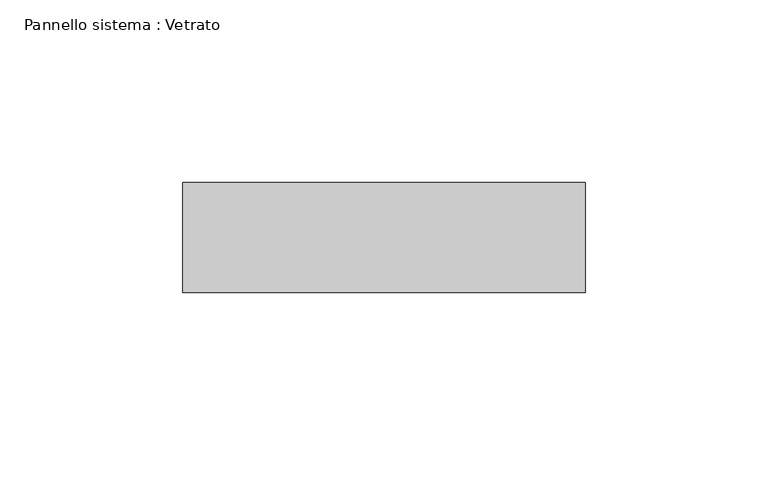
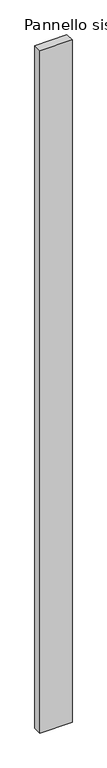
"""IFC4 building model written with IfcOpenShell, lengths in millimetres: plate geometry, Pannello sistema : Vetrato."""

from ifc_helpers import new_model, si_unit, origin, origin_with_axes, place, context, project, spatial, polyline, outline, extrude, source, transform, mapped, element, save


def pannello_sistema_vetrato_b6e2c1f0(model_context):
    return source(origin(), model_context, "Body", "SweptSolid", [
        extrude(outline(polyline([(55.0, -15.0), (-55.0, -15.0), (-55.0, 15.0), (55.0, 15.0), (55.0, -15.0)])), origin_with_axes(), (0.0, 0.0, 1.0), 2475.0),
    ])


if __name__ == "__main__":
    model = new_model("IFC4")
    model_context = context("Model", 3, world=origin())
    ifc_project = project(units=[si_unit("LENGTHUNIT", "METRE", prefix="MILLI")], contexts=[model_context])
    site = spatial("IfcSite", under=ifc_project)
    building = spatial("IfcBuilding", under=site)
    placement = place(None, origin())
    pannello_sistema_vetrato_shape = pannello_sistema_vetrato_b6e2c1f0(model_context)
    element("IfcPlate", 1, ObjectType="Pannello sistema : Vetrato", at=placement, inside=building, context=model_context, shape_type="MappedRepresentation", body=[
        mapped(pannello_sistema_vetrato_shape, transform((0.0, 0.0, 0.0), x_axis=(1.0, 0.0, 0.0), y_axis=(0.0, 1.0, 0.0), z_axis=(0.0, 0.0, 1.0))),
    ])
    save(model, "model.ifc")

# Revit data of these elements
# Type "Pannello sistema : Vetrato"
#   Construction Type Id = "GSP4R"
#   Analytic Construction = "Vetrata singola Pilkington 1/8 in"
#   Visual Light Transmittance = 0.9
#   Solar Heat Gain Coefficient = 0.86
#   Heat Transfer Coefficient (U) = 6.7069 W/(m²·K)
# Element 1 (IfcPlate, "Pannello sistema : Vetrato")
#   Materials on its faces: "Default - Vetro"
# Materials
#   "Default - Vetro": class "Vetro", colour RGB 208 208 208, transparency 0.7, Cost = 0
